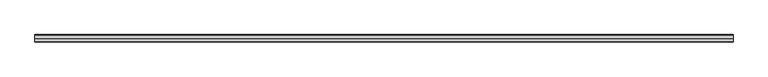
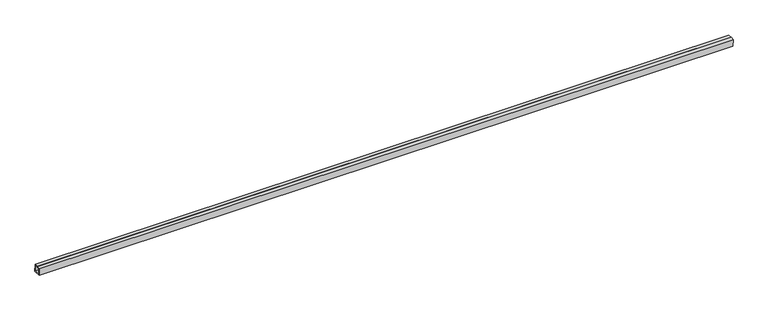
"""IFC4 building model written with IfcOpenShell, lengths in millimetres: proxy geometry, Inner panel:Inner panel:1:Inner panel:1 : Inner panel:Inner panel:300324:2:Inner panel:1:Inner panel:1 : Inner panel:Inner panel:300324:2 : Inner panel:Inner panel:1:Inner panel:1 : Inner panel:Inner panel:300324:300043:48 : Inner panel:Inner panel:1:Inner panel:1 : Inner panel:Inner panel:300324:2:Inner panel:1:Inner panel:1 : Inner panel:Inner panel:300324:2 : Inner panel:Inner panel:1:Inner panel:1 : Inner panel:Inner panel:300324:300043:308120."""

from ifc_helpers import new_model, si_unit, frame, origin, place, context, project, spatial, polyline, outline, extrude, source, transform, mapped, element, save


def generic_models_4139b04b(model_context):
    return source(origin(), model_context, "Body", "SweptSolid", [
        extrude(outline(polyline([(-581211.0091179, 3857.8017792), (-581192.7686948, 3858.5617968), (-581191.182571, 3820.4948267), (-581229.2495411, 3818.908703), (-581230.8356649, 3856.9756731), (-581212.5952417, 3857.7356907), (-581212.496109, 3855.3565051), (-581228.3573465, 3854.6956202), (-581226.9694882, 3821.3870213), (-581193.6608894, 3822.7748796), (-581195.0487477, 3856.0834785), (-581210.9099852, 3855.4225936), (-581211.0091179, 3857.8017792)])), frame((664223.0867238, 0.0, 0.0), z_axis=(1.0, 0.0, 0.0), x_axis=(0.0, 1.0, 0.0)), (0.0, 0.0, 1.0), 3657.6),
    ])


if __name__ == "__main__":
    model = new_model("IFC4")
    model_context = context("Model", 3, world=origin())
    ifc_project = project(units=[si_unit("LENGTHUNIT", "METRE", prefix="MILLI")], contexts=[model_context])
    site = spatial("IfcSite", under=ifc_project)
    building = spatial("IfcBuilding", under=site)
    placement = place(None, origin())
    generic_models_shape = generic_models_4139b04b(model_context)
    element("IfcBuildingElementProxy", 1, Name="Inner panel:Inner panel:1:Inner panel:1 : Inner panel:Inner panel:300324:2:Inner panel:1:Inner panel:1 : Inner panel:Inner panel:300324:2 : Inner panel:Inner panel:1:Inner panel:1 : Inner panel:Inner panel:300324:300043:48 : Inner panel:Inner panel:1:Inner panel:1 : Inner panel:Inner panel:300324:2:Inner panel:1:Inner panel:1 : Inner panel:Inner panel:300324:2 : Inner panel:Inner panel:1:Inner panel:1 : Inner panel:Inner panel:300324:300043:308120", ObjectType="Inner panel:Inner panel:1:Inner panel:1 : Inner panel:Inner panel:300324:2:Inner panel:1:Inner panel:1 : Inner panel:Inner panel:300324:2 : Inner panel:Inner panel:1:Inner panel:1 : Inner panel:Inner panel:300324:300043:48 : Inner panel:Inner panel:1:Inner panel:1 : Inner panel:Inner panel:300324:2:Inner panel:1:Inner panel:1 : Inner panel:Inner panel:300324:2 : Inner panel:Inner panel:1:Inner panel:1 : Inner panel:Inner panel:300324:300043:308120", at=placement, inside=building, context=model_context, shape_type="MappedRepresentation", body=[
        mapped(generic_models_shape, transform((0.0, 0.0, 0.0), x_axis=(1.0, 0.0, 0.0), y_axis=(0.0, 1.0, 0.0), z_axis=(0.0, 0.0, 1.0))),
    ])
    save(model, "model.ifc")

# Revit data of these elements
# Type "Inner panel:Inner panel:1:Inner panel:1 : Inner panel:Inner panel:300324:2:Inner panel:1:Inner panel:1 : Inner panel:Inner panel:300324:2 : Inner panel:Inner panel:1:Inner panel:1 : Inner panel:Inner panel:300324:300043:48 : Inner panel:Inner panel:1:Inner panel:1 : Inner panel:Inner panel:300324:2:Inner panel:1:Inner panel:1 : Inner panel:Inner panel:300324:2 : Inner panel:Inner panel:1:Inner panel:1 : Inner panel:Inner panel:300324:300043:308120"
#   NameOverride = "Inner panel:Inner panel:1:Inner panel:1 : Inner panel:Inner panel:300324:2:Inner panel:1:Inner panel:1 : Inner panel:Inner panel:300324:2 : Inner panel:Inner panel:1:Inner panel:1 : Inner panel:Inner panel:300324:300043:308120"
#   ObjectTypeOverride = "Inner panel:1:Inner panel:1 : Inner panel:Inner panel:300324:2 : Inner panel:Inner panel:1:Inner panel:1 : Inner panel:Inner panel:300324:300043"
#   Reference = "Inner panel"
#   Tag = "308120"
# Element 1 (IfcBuildingElementProxy, "Inner panel:Inner panel:1:Inner panel:1 : Inner panel:Inner panel:300324:2:Inner panel:1:Inner panel:1 : Inner panel:Inner panel:300324:2 : Inner panel:Inner panel:1:Inner panel:1 : Inner panel:Inner panel:300324:300043:48 : Inner panel:Inner panel:1:Inner panel:1 : Inner panel:Inner panel:300324:2:Inner panel:1:Inner panel:1 : Inner panel:Inner panel:300324:2 : Inner panel:Inner panel:1:Inner panel:1 : Inner panel:Inner panel:300324:300043:308120")
#   Materials on its faces: "1 1/2\" X 1 1/2\" SPLIT-SEAM SQUARE TUBING (~24\" CANTILEVER FROM C.L. OF GLULAM)"
# Materials
#   "1 1/2\" X 1 1/2\" SPLIT-SEAM SQUARE TUBING (~24\" CANTILEVER FROM C.L. OF GLULAM)": class "Unassigned", colour RGB 202 201 200, transparency 0, Cost = 0
